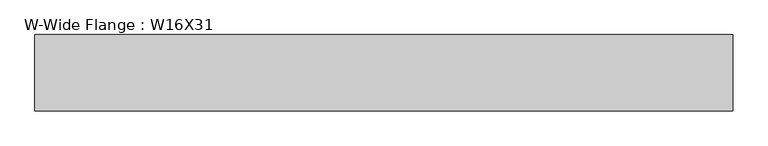
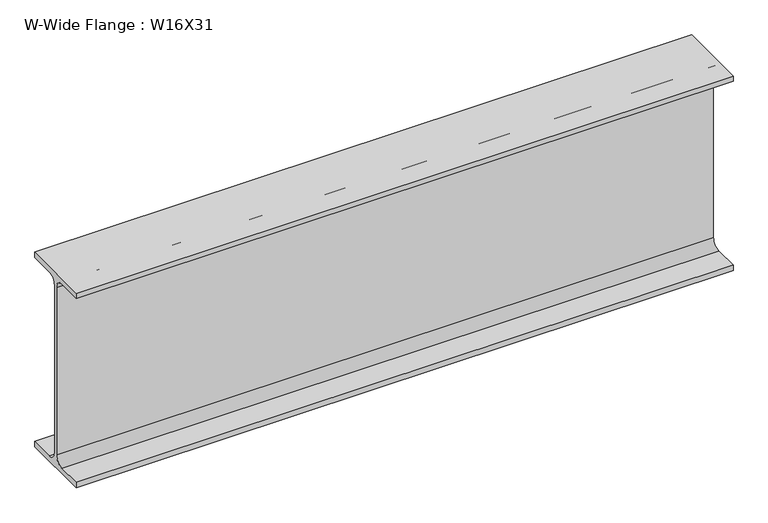
"""IFC4 building model written with IfcOpenShell, lengths in millimetres: beam geometry, W-Wide Flange : W16X31."""

from ifc_helpers import new_model, si_unit, point, frame, frame_2d, origin, place, context, project, spatial, polyline, circle_curve, trimmed, segment, composite_curve, outline, extrude, source, transform, mapped, element, save


def w_wide_flange_w16x31_4661288e(model_context):
    return source(origin(), model_context, "Body", "SweptSolid", [
        extrude(outline(composite_curve([segment(polyline([(70.231, -190.754), (70.231, -201.93), (-70.231, -201.93), (-70.231, -190.754), (-20.8915, -190.754)]), True, "CONTINUOUS"), segment(trimmed(circle_curve(frame_2d((-20.8915, -173.355)), 17.399), [point((-20.8915, -190.754))], [point((-3.4925, -173.355))], True, "CARTESIAN"), True, "CONTINUOUS"), segment(polyline([(-3.4925, -173.355), (-3.4925, 173.355)]), True, "CONTINUOUS"), segment(trimmed(circle_curve(frame_2d((-20.8915, 173.355)), 17.399), [point((-3.4925, 173.355))], [point((-20.8915, 190.754))], True, "CARTESIAN"), True, "CONTINUOUS"), segment(polyline([(-20.8915, 190.754), (-70.231, 190.754), (-70.231, 201.93), (70.231, 201.93), (70.231, 190.754), (20.8915, 190.754)]), True, "CONTINUOUS"), segment(trimmed(circle_curve(frame_2d((20.8915, 173.355)), 17.399), [point((20.8915, 190.754))], [point((3.4925, 173.355))], True, "CARTESIAN"), True, "CONTINUOUS"), segment(polyline([(3.4925, 173.355), (3.4925, -173.355)]), True, "CONTINUOUS"), segment(trimmed(circle_curve(frame_2d((20.8915, -173.355)), 17.399), [point((3.4925, -173.355))], [point((20.8915, -190.754))], True, "CARTESIAN"), True, "CONTINUOUS"), segment(polyline([(20.8915, -190.754), (70.231, -190.754)]), True, "CONTINUOUS")], self_intersect=False)), frame((-580.2981568, 0.0, 0.0), z_axis=(1.0, 0.0, 0.0), x_axis=(0.0, 1.0, 0.0)), (0.0, 0.0, 1.0), 1287.5963136),
    ])


if __name__ == "__main__":
    model = new_model("IFC4")
    model_context = context("Model", 3, world=origin())
    ifc_project = project(units=[si_unit("LENGTHUNIT", "METRE", prefix="MILLI")], contexts=[model_context])
    site = spatial("IfcSite", under=ifc_project)
    building = spatial("IfcBuilding", under=site)
    placement = place(None, origin())
    w_wide_flange_w16x31_shape = w_wide_flange_w16x31_4661288e(model_context)
    element("IfcBeam", 1, ObjectType="W-Wide Flange : W16X31", at=placement, inside=building, context=model_context, shape_type="MappedRepresentation", body=[
        mapped(w_wide_flange_w16x31_shape, transform((0.0, 0.0, 0.0), x_axis=(1.0, 0.0, 0.0), y_axis=(0.0, 1.0, 0.0), z_axis=(0.0, 0.0, 1.0))),
    ])
    save(model, "model.ifc")

# Revit data of these elements
# Type "W-Wide Flange : W16X31"
#   Assembly Code = "B10"
#   W = 31
#   Length [instance default] = 5' - 0"
#   bf = 0' - 5.53"
#   d = 1' - 3.9"
#   k = 0' - 1 1/8"
#   k2 = 0' - 0.685"
#   tf = 0' - 0.44"
#   tw = 0' - 0.275"
#   A = 0.0634028 SF
#   Structural Material [instance default] = Steel ASTM A992
# Element 1 (IfcBeam, "W-Wide Flange : W16X31")
#   Materials on its faces: "Steel ASTM A992"
# Materials
#   "Steel ASTM A992": class "Metal", colour RGB 199 199 199, transparency 0, Description = "Structural steel 50ksi", Cost = 0
